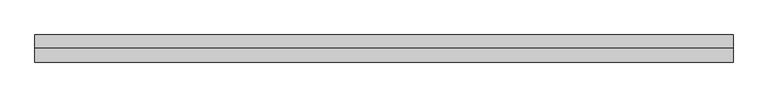
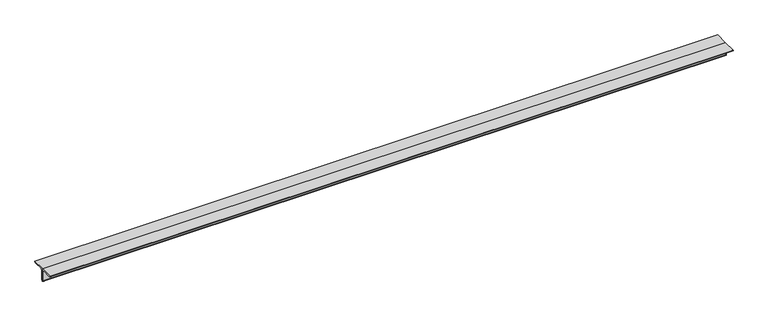
"""IFC4 building model written with IfcOpenShell, lengths in millimetres: member geometry, Steel Framing_2Ls_KS : H_SB_AR_S02_2Ls-100x100x10_VBR1."""

from ifc_helpers import new_model, si_unit, point, frame, frame_2d, origin, place, context, project, spatial, polyline, circle_curve, trimmed, segment, composite_curve, outline, extrude, source, transform, mapped, element, save


def member_c1cadd4c(model_context):
    return source(origin(), model_context, "Body", "SweptSolid", [
        extrude(outline(composite_curve([segment(polyline([(0.0, 28.2), (0.0, -71.8)]), True, "CONTINUOUS"), segment(trimmed(circle_curve(frame_2d((0.0, -61.8)), 10.0), [point((0.0, -71.8))], [point((-10.0, -61.8))], False, "CARTESIAN"), True, "CONTINUOUS"), segment(polyline([(-10.0, -61.8), (-10.0, 8.2)]), True, "CONTINUOUS"), segment(trimmed(circle_curve(frame_2d((-20.0, 8.2)), 10.0), [point((-10.0, 8.2))], [point((-20.0, 18.2))], True, "CARTESIAN"), True, "CONTINUOUS"), segment(polyline([(-20.0, 18.2), (-90.0, 18.2)]), True, "CONTINUOUS"), segment(trimmed(circle_curve(frame_2d((-90.0, 28.2)), 10.0), [point((-90.0, 18.2))], [point((-100.0, 28.2))], False, "CARTESIAN"), True, "CONTINUOUS"), segment(polyline([(-100.0, 28.2), (0.0, 28.2)]), True, "CONTINUOUS")], self_intersect=False)), frame((-2600.492603, 0.0, 0.0), z_axis=(1.0, 0.0, 0.0), x_axis=(0.0, 1.0, 0.0)), (0.0, 0.0, 1.0), 5152.5727888),
        extrude(outline(composite_curve([segment(polyline([(0.0, 28.2), (100.0, 28.2)]), True, "CONTINUOUS"), segment(trimmed(circle_curve(frame_2d((90.0, 28.2)), 10.0), [point((100.0, 28.2))], [point((90.0, 18.2))], False, "CARTESIAN"), True, "CONTINUOUS"), segment(polyline([(90.0, 18.2), (20.0, 18.2)]), True, "CONTINUOUS"), segment(trimmed(circle_curve(frame_2d((20.0, 8.2)), 10.0), [point((20.0, 18.2))], [point((10.0, 8.2))], True, "CARTESIAN"), True, "CONTINUOUS"), segment(polyline([(10.0, 8.2), (10.0, -61.8)]), True, "CONTINUOUS"), segment(trimmed(circle_curve(frame_2d((0.0, -61.8)), 10.0), [point((10.0, -61.8))], [point((0.0, -71.8))], False, "CARTESIAN"), True, "CONTINUOUS"), segment(polyline([(0.0, -71.8), (0.0, 28.2)]), True, "CONTINUOUS")], self_intersect=False)), frame((-2600.492603, 0.0, 0.0), z_axis=(1.0, 0.0, 0.0), x_axis=(0.0, 1.0, 0.0)), (0.0, 0.0, 1.0), 5152.5727888),
    ])


if __name__ == "__main__":
    model = new_model("IFC4")
    model_context = context("Model", 3, world=origin())
    ifc_project = project(units=[si_unit("LENGTHUNIT", "METRE", prefix="MILLI")], contexts=[model_context])
    site = spatial("IfcSite", under=ifc_project)
    building = spatial("IfcBuilding", under=site)
    placement = place(None, origin())
    member_shape = member_c1cadd4c(model_context)
    element("IfcMember", 1, ObjectType="Steel Framing_2Ls_KS : H_SB_AR_S02_2Ls-100x100x10_VBR1", at=placement, inside=building, context=model_context, shape_type="MappedRepresentation", body=[
        mapped(member_shape, transform((0.0, 0.0, 0.0), x_axis=(1.0, 0.0, 0.0), y_axis=(0.0, 1.0, 0.0), z_axis=(0.0, 0.0, 1.0))),
    ])
    save(model, "model.ifc")

# Revit data of these elements
# Type "Steel Framing_2Ls_KS : H_SB_AR_S02_2Ls-100x100x10_VBR1"
#   Type Comments = "MAIN"
#   Type Mark = "VBR1"
#   H_SectionID = "2Ls-100x100x10"
#   Assembly Code = "B10"
#   Legs = "LLBB"
#   H_Ratio for Additional Steel Plate = 0.2
#   W = 0
#   Perimeter = 0.80 m²/m
#   Nominal Weight = 29.80 kgf/m
#   Length [instance default] = 1524 mm
#   Space = 0 mm
#   b = 100 mm
#   d = 100 mm
#   t = 10 mm
#   y = 28.2 mm
#   A = 0.0038 m²
#   Structural Material [instance default] = Steel, 45-345
# Element 1 (IfcMember, "Steel Framing_2Ls_KS : H_SB_AR_S02_2Ls-100x100x10_VBR1")
#   Materials on its faces: "Steel, 45-345"
# Materials
#   "Steel, 45-345": class "Metal", colour RGB 189 187 185, transparency 0, Description = "Steel 345 MPa", Cost = 0
